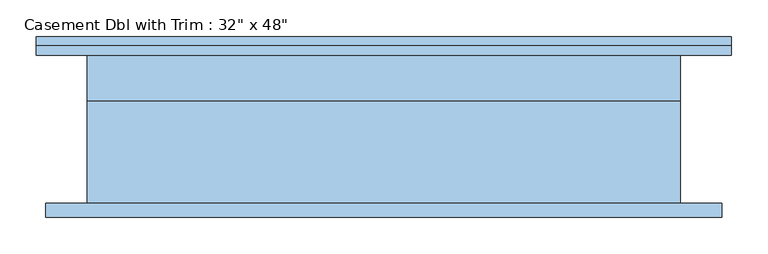
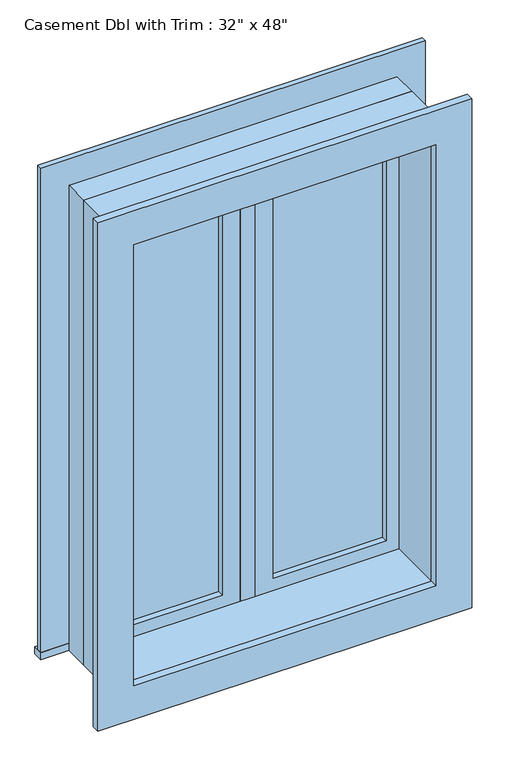
"""IFC4 building model written with IfcOpenShell, lengths in millimetres: window geometry."""

import ifcopenshell
import ifcopenshell.guid

model = None  # the IFC model being written
_history = None  # IfcOwnerHistory: only IFC2X3 demands one
_inside = {}  # id of a spatial element -> (the spatial element, [elements in it])
_under = {}  # id of a project, library or spatial element -> (it, [spatial elements below it])
_declared = {}  # id of a project -> (the project, [libraries it declares])
_typed = {}  # id of a type object -> (the type object, [elements of that type])
_made_of = {}  # id of a material, layer set ... -> (it, [elements and type objects made of it])


def new_model(schema):
    """Start an empty IFC model of exactly this schema.

    Asked for "IFC4X3", IfcOpenShell would pick the latest addendum, in which some entities
    have other attributes; the version numbers below select the first issue.
    IFC2X3 requires an IfcOwnerHistory on every rooted entity: one is made here for all.
    """
    global model, _history
    if schema == "IFC4X3":
        model = ifcopenshell.file(schema_version=(4, 3, 0, 0))
    else:
        model = ifcopenshell.file(schema=schema)
    _inside.clear()
    _under.clear()
    _declared.clear()
    _typed.clear()
    _made_of.clear()
    _history = None
    if model.schema == "IFC2X3":
        org = make("IfcOrganization", Name="unknown")
        user = make(
            "IfcPersonAndOrganization",
            ThePerson=make("IfcPerson", FamilyName="unknown"),
            TheOrganization=org,
        )
        app = make(
            "IfcApplication",
            ApplicationDeveloper=org,
            Version="unknown",
            ApplicationFullName="unknown",
            ApplicationIdentifier="unknown",
        )
        _history = make(
            "IfcOwnerHistory",
            OwningUser=user,
            OwningApplication=app,
            ChangeAction="ADDED",
            CreationDate=0,
        )
    return model


def make(cls, **values):
    """One entity of the class cls with the attributes given. An attribute that is None is left unset."""
    return model.create_entity(
        cls, **{name: value for name, value in values.items() if value is not None}
    )


def rooted(cls, **values):
    """An entity with a GlobalId (a new one), such as an element, a storey or a relation."""
    return make(cls, GlobalId=ifcopenshell.guid.new(), OwnerHistory=_history, **values)


def si_unit(unit_type, name, prefix=None):
    """IfcSIUnit, for example si_unit("LENGTHUNIT", "METRE", prefix="MILLI")."""
    return make("IfcSIUnit", UnitType=unit_type, Prefix=prefix, Name=name)


def assignment(units):
    """IfcUnitAssignment: the units of a project."""
    return None if units is None else make("IfcUnitAssignment", Units=units)


def point(xyz):
    """IfcCartesianPoint."""
    return None if xyz is None else make("IfcCartesianPoint", Coordinates=xyz)


def direction(xyz):
    """IfcDirection."""
    return None if xyz is None else make("IfcDirection", DirectionRatios=xyz)


def frame(location, z_axis=None, x_axis=None):
    """IfcAxis2Placement3D, a coordinate frame: its origin and axes. An axis left out is left unset."""
    return make(
        "IfcAxis2Placement3D",
        Location=point(location),
        Axis=direction(z_axis),
        RefDirection=direction(x_axis),
    )


def origin():
    """The frame at (0, 0, 0) with its axes left unset."""
    return frame((0.0, 0.0, 0.0))


def place(relative_to, where):
    """IfcLocalPlacement: puts the frame where relative to a parent placement (None: the world)."""
    return make(
        "IfcLocalPlacement", PlacementRelTo=relative_to, RelativePlacement=where
    )


def context(
    kind, dimensions, precision=None, world=None, true_north=None, identifier=None
):
    """IfcGeometricRepresentationContext, for example the 3D "Model" context."""
    return make(
        "IfcGeometricRepresentationContext",
        ContextIdentifier=identifier,
        ContextType=kind,
        CoordinateSpaceDimension=dimensions,
        Precision=precision,
        WorldCoordinateSystem=world,
        TrueNorth=true_north,
    )


def project(units=None, contexts=None):
    """IfcProject with its units and contexts."""
    return rooted(
        "IfcProject",
        Name="project",
        RepresentationContexts=contexts,
        UnitsInContext=assignment(units),
    )


def spatial(cls, under=None, at=None, **own):
    """A site, building, storey or space (cls), placed at a placement, below another one or the project."""
    s = rooted(cls, ObjectPlacement=at, **own)
    if under is not None:
        _under.setdefault(under.id(), (under, []))[1].append(s)
    return s


def polyline(points):
    """IfcPolyline through the points."""
    return make("IfcPolyline", Points=[point(p) for p in points])


def outline(outer, holes=None, kind="AREA"):
    """IfcArbitraryClosedProfileDef: a profile drawn as a closed curve; with holes, ...WithVoids."""
    if holes is None:
        return make("IfcArbitraryClosedProfileDef", ProfileType=kind, OuterCurve=outer)
    return make(
        "IfcArbitraryProfileDefWithVoids",
        ProfileType=kind,
        OuterCurve=outer,
        InnerCurves=holes,
    )


def extrude(swept, where, along, depth):
    """IfcExtrudedAreaSolid: the profile swept, set in the frame where, extruded along a direction by depth."""
    return make(
        "IfcExtrudedAreaSolid",
        SweptArea=swept,
        Position=where,
        ExtrudedDirection=direction(along),
        Depth=depth,
    )


def shape(context_of_items, identifier, shape_type, items):
    """IfcShapeRepresentation: the items that make up one representation, for example the "Body"."""
    return make(
        "IfcShapeRepresentation",
        ContextOfItems=context_of_items,
        RepresentationIdentifier=identifier,
        RepresentationType=shape_type,
        Items=items,
    )


def source(mapping_origin, context_of_items, identifier, shape_type, items):
    """IfcRepresentationMap: a shape defined once, which mapped items show again and again."""
    return make(
        "IfcRepresentationMap",
        MappingOrigin=mapping_origin,
        MappedRepresentation=shape(context_of_items, identifier, shape_type, items),
    )


def transform(
    local_origin,
    x_axis=None,
    y_axis=None,
    z_axis=None,
    scale=None,
    scale2=None,
    scale3=None,
    uniform=True,
):
    """IfcCartesianTransformationOperator3D, or its non-uniform kind. x_axis, y_axis, z_axis: its Axis1, 2, 3."""
    if uniform:
        return make(
            "IfcCartesianTransformationOperator3D",
            Axis1=direction(x_axis),
            Axis2=direction(y_axis),
            LocalOrigin=point(local_origin),
            Scale=scale,
            Axis3=direction(z_axis),
        )
    return make(
        "IfcCartesianTransformationOperator3DnonUniform",
        Axis1=direction(x_axis),
        Axis2=direction(y_axis),
        LocalOrigin=point(local_origin),
        Scale=scale,
        Axis3=direction(z_axis),
        Scale2=scale2,
        Scale3=scale3,
    )


def mapped(mapping_source, mapping_target):
    """IfcMappedItem: shows the shape of a source again, moved by a transform."""
    return make(
        "IfcMappedItem", MappingSource=mapping_source, MappingTarget=mapping_target
    )


def made_of(thing, what):
    """Note that an element or type object is made of a material, layer set ...; save() writes the relation."""
    if what is not None:
        _made_of.setdefault(what.id(), (what, []))[1].append(thing)
    return thing


def element(
    cls,
    number,
    at=None,
    inside=None,
    cuts=None,
    type_object=None,
    material=None,
    context=None,
    identifier="Body",
    shape_type=None,
    held_by="IfcProductDefinitionShape",
    body=None,
    shapes=None,
    **own,
):
    """One element of the class cls, such as IfcWall. Its Tag is "e" and its number.

    at: its placement. inside: the storey or other place that contains it. cuts: it is an
    opening in that element (IfcRelVoidsElement). A single representation is given by context,
    identifier, shape_type and body (its items); several are given by shapes. held_by: the class
    of the entity that holds the representations. save() writes the other relations.
    """
    e = rooted(cls, Tag="e%d" % number, ObjectPlacement=at, **own)
    if body is not None:
        shapes = [shape(context, identifier, shape_type, body)]
    if shapes is not None:
        e.Representation = make(held_by, Representations=shapes)
    if inside is not None:
        _inside.setdefault(inside.id(), (inside, []))[1].append(e)
    if cuts is not None:
        rooted(
            "IfcRelVoidsElement", RelatingBuildingElement=cuts, RelatedOpeningElement=e
        )
    if type_object is not None:
        _typed.setdefault(type_object.id(), (type_object, []))[1].append(e)
    return made_of(e, material)


def aggregate(whole, parts):
    """IfcRelAggregates: a whole, such as a stair, and the parts it consists of."""
    return rooted("IfcRelAggregates", RelatingObject=whole, RelatedObjects=parts)


def save(model, path):
    """Write the relations noted so far, then the file.

    IfcRelAggregates (storeys below a building ...), IfcRelContainedInSpatialStructure (elements
    in a storey), IfcRelDefinesByType, IfcRelAssociatesMaterial and IfcRelDeclares: one each for
    every whole, place, type object, material and project.
    """
    for whole, parts in _under.values():
        aggregate(whole, parts)
    for where, things in _inside.values():
        rooted(
            "IfcRelContainedInSpatialStructure",
            RelatedElements=things,
            RelatingStructure=where,
        )
    for kind, things in _typed.values():
        rooted("IfcRelDefinesByType", RelatedObjects=things, RelatingType=kind)
    for what, things in _made_of.values():
        rooted("IfcRelAssociatesMaterial", RelatedObjects=things, RelatingMaterial=what)
    for by, libraries in _declared.values():
        rooted("IfcRelDeclares", RelatingContext=by, RelatedDefinitions=libraries)
    model.write(path)


def window_bb17773d(model_context):
    return source(origin(), model_context, "Body", "SweptSolid", [
        extrude(outline(polyline([(63.5, 85.725), (342.9, 85.725), (342.9, 73.025), (63.5, 73.025), (63.5, 85.725)])), frame((0.0, 0.0, 977.9), z_axis=(0.0, 0.0, 1.0), x_axis=(1.0, 0.0, 0.0)), (0.0, 0.0, 1.0), 1092.2),
        extrude(outline(polyline([(2114.55, 19.05), (933.45, 19.05), (933.45, 387.35), (2114.55, 387.35), (2114.55, 19.05)]), holes=[polyline([(2070.1, 63.5), (2070.1, 342.9), (977.9, 342.9), (977.9, 63.5), (2070.1, 63.5)])]), frame((0.0, 57.15, 0.0), z_axis=(0.0, 1.0, 0.0), x_axis=(0.0, 0.0, 1.0)), (0.0, 0.0, 1.0), 44.45),
        extrude(outline(polyline([(19.05, 57.15), (-19.05, 57.15), (-19.05, 120.65), (19.05, 120.65), (19.05, 57.15)])), frame((0.0, 0.0, 933.45), z_axis=(0.0, 0.0, 1.0), x_axis=(1.0, 0.0, 0.0)), (0.0, 0.0, 1.0), 1181.1),
        extrude(outline(polyline([(-476.25, 146.05), (476.25, 146.05), (476.25, 120.65), (-476.25, 120.65), (-476.25, 146.05)])), frame((0.0, 0.0, 914.4), z_axis=(0.0, 0.0, 1.0), x_axis=(1.0, 0.0, 0.0)), (0.0, 0.0, 1.0), 19.05),
        extrude(outline(polyline([(2114.55, -387.35), (2114.55, 387.35), (933.45, 387.35), (933.45, 476.25), (2203.45, 476.25), (2203.45, -476.25), (933.45, -476.25), (933.45, -387.35), (2114.55, -387.35)])), frame((0.0, 120.65, 0.0), z_axis=(0.0, 1.0, 0.0), x_axis=(0.0, 0.0, 1.0)), (0.0, 0.0, 1.0), 12.7),
        extrude(outline(polyline([(2190.75, 463.55), (2190.75, -463.55), (857.25, -463.55), (857.25, 463.55), (2190.75, 463.55)]), holes=[polyline([(2101.85, 374.65), (946.15, 374.65), (946.15, -374.65), (2101.85, -374.65), (2101.85, 374.65)])]), frame((0.0, -101.6, 0.0), z_axis=(0.0, 1.0, 0.0), x_axis=(0.0, 0.0, 1.0)), (0.0, 0.0, 1.0), 19.05),
        extrude(outline(polyline([(-63.5, 73.025), (-342.9, 73.025), (-342.9, 85.725), (-63.5, 85.725), (-63.5, 73.025)])), frame((0.0, 0.0, 977.9), z_axis=(0.0, 0.0, 1.0), x_axis=(1.0, 0.0, 0.0)), (0.0, 0.0, 1.0), 1092.2),
        extrude(outline(polyline([(2114.55, -387.35), (933.45, -387.35), (933.45, -19.05), (2114.55, -19.05), (2114.55, -387.35)]), holes=[polyline([(2070.1, -342.9), (2070.1, -63.5), (977.9, -63.5), (977.9, -342.9), (2070.1, -342.9)])]), frame((0.0, 57.15, 0.0), z_axis=(0.0, 1.0, 0.0), x_axis=(0.0, 0.0, 1.0)), (0.0, 0.0, 1.0), 44.45),
        extrude(outline(polyline([(2133.6, -406.4), (914.4, -406.4), (914.4, 406.4), (2133.6, 406.4), (2133.6, -406.4)]), holes=[polyline([(2101.85, -374.65), (2101.85, 374.65), (946.15, 374.65), (946.15, -374.65), (2101.85, -374.65)])]), frame((0.0, -82.55, 0.0), z_axis=(0.0, 1.0, 0.0), x_axis=(0.0, 0.0, 1.0)), (0.0, 0.0, 1.0), 139.7),
        extrude(outline(polyline([(2133.6, 406.4), (2133.6, -406.4), (914.4, -406.4), (914.4, 406.4), (2133.6, 406.4)]), holes=[polyline([(2114.55, 387.35), (933.45, 387.35), (933.45, -387.35), (2114.55, -387.35), (2114.55, 387.35)])]), frame((0.0, 57.15, 0.0), z_axis=(0.0, 1.0, 0.0), x_axis=(0.0, 0.0, 1.0)), (0.0, 0.0, 1.0), 63.5),
    ])


if __name__ == "__main__":
    model = new_model("IFC4")
    model_context = context("Model", 3, world=origin())
    ifc_project = project(units=[si_unit("LENGTHUNIT", "METRE", prefix="MILLI")], contexts=[model_context])
    site = spatial("IfcSite", under=ifc_project)
    building = spatial("IfcBuilding", under=site)
    placement = place(None, origin())
    window_shape = window_bb17773d(model_context)
    element("IfcWindow", 1, ObjectType="Casement Dbl with Trim : 32\" x 48\"", at=placement, inside=building, context=model_context, shape_type="MappedRepresentation", body=[
        mapped(window_shape, transform((0.0, 0.0, 0.0), x_axis=(1.0, 0.0, 0.0), y_axis=(0.0, 1.0, 0.0), z_axis=(0.0, 0.0, 1.0))),
    ])
    save(model, "model.ifc")

# Revit data of these elements
# Type "Casement Dbl with Trim : 32\" x 48\""
#   Type Mark = "12"
#   Construction Type Id = "GSP4R"
#   Assembly Code = "B2020100"
#   Analytic Construction = "1/8 in Pilkington single glazing"
#   Visual Light Transmittance = 0.9
#   Solar Heat Gain Coefficient = 0.78
#   Heat Transfer Coefficient (U) = 3.6886 W/(m²·K)
#   Height = 4' - 0"
#   Default Sill Height = 3' - 0"
#   Trim Projection - Ext. = 0' - 0 1/2"
#   Trim Projection - Int. = 0' - 0 3/4"
#   Trim Width - Exterior = 0' - 3 1/2"
#   Trim Width - Interior = 0' - 3 1/2"
#   Width = 2' - 8"
#   Window Inset = 0' - 0 3/4"
#   Glass Pane Material = Glass
#   Sash Material = Sash
#   Trim Exterior Material = Trim
#   Trim Interior Material = Trim
#   Wall Closure = (empty or 0)
# Element 1 (IfcWindow, "Casement Dbl with Trim : 32\" x 48\"")
#   Materials on its faces: "Sash", "Trim", "Glass"
# Materials
#   "Glass": class "Glass", colour RGB 0 128 192, transparency 0.75, Description = "Soda Lime Glass", Cost = 0
#   "Sash": class "Wood", colour RGB 224 178 126, transparency 0, Cost = 0
#   "Trim": class "Wood", colour RGB 224 178 126, transparency 0
